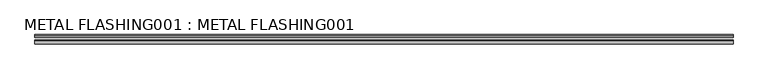
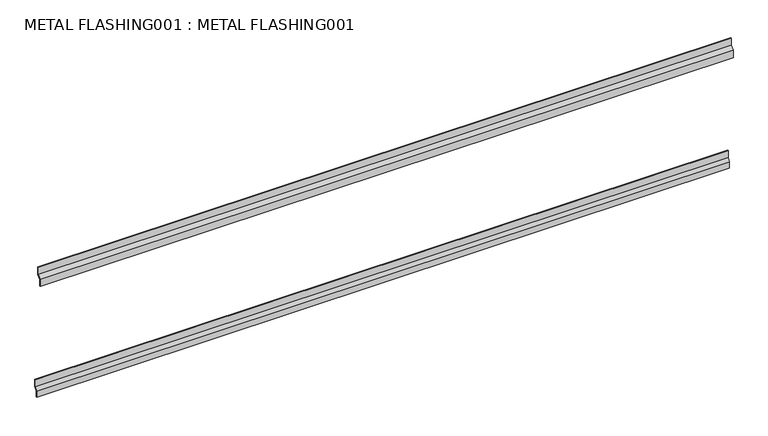
"""IFC4 building model written with IfcOpenShell, lengths in millimetres: proxy geometry, METAL FLASHING001 : METAL FLASHING001."""

import ifcopenshell
import ifcopenshell.guid

model = None  # the IFC model being written
_history = None  # IfcOwnerHistory: only IFC2X3 demands one
_inside = {}  # id of a spatial element -> (the spatial element, [elements in it])
_under = {}  # id of a project, library or spatial element -> (it, [spatial elements below it])
_declared = {}  # id of a project -> (the project, [libraries it declares])
_typed = {}  # id of a type object -> (the type object, [elements of that type])
_made_of = {}  # id of a material, layer set ... -> (it, [elements and type objects made of it])


def new_model(schema):
    """Start an empty IFC model of exactly this schema.

    Asked for "IFC4X3", IfcOpenShell would pick the latest addendum, in which some entities
    have other attributes; the version numbers below select the first issue.
    IFC2X3 requires an IfcOwnerHistory on every rooted entity: one is made here for all.
    """
    global model, _history
    if schema == "IFC4X3":
        model = ifcopenshell.file(schema_version=(4, 3, 0, 0))
    else:
        model = ifcopenshell.file(schema=schema)
    _inside.clear()
    _under.clear()
    _declared.clear()
    _typed.clear()
    _made_of.clear()
    _history = None
    if model.schema == "IFC2X3":
        org = make("IfcOrganization", Name="unknown")
        user = make(
            "IfcPersonAndOrganization",
            ThePerson=make("IfcPerson", FamilyName="unknown"),
            TheOrganization=org,
        )
        app = make(
            "IfcApplication",
            ApplicationDeveloper=org,
            Version="unknown",
            ApplicationFullName="unknown",
            ApplicationIdentifier="unknown",
        )
        _history = make(
            "IfcOwnerHistory",
            OwningUser=user,
            OwningApplication=app,
            ChangeAction="ADDED",
            CreationDate=0,
        )
    return model


def make(cls, **values):
    """One entity of the class cls with the attributes given. An attribute that is None is left unset."""
    return model.create_entity(
        cls, **{name: value for name, value in values.items() if value is not None}
    )


def rooted(cls, **values):
    """An entity with a GlobalId (a new one), such as an element, a storey or a relation."""
    return make(cls, GlobalId=ifcopenshell.guid.new(), OwnerHistory=_history, **values)


def si_unit(unit_type, name, prefix=None):
    """IfcSIUnit, for example si_unit("LENGTHUNIT", "METRE", prefix="MILLI")."""
    return make("IfcSIUnit", UnitType=unit_type, Prefix=prefix, Name=name)


def assignment(units):
    """IfcUnitAssignment: the units of a project."""
    return None if units is None else make("IfcUnitAssignment", Units=units)


def point(xyz):
    """IfcCartesianPoint."""
    return None if xyz is None else make("IfcCartesianPoint", Coordinates=xyz)


def direction(xyz):
    """IfcDirection."""
    return None if xyz is None else make("IfcDirection", DirectionRatios=xyz)


def frame(location, z_axis=None, x_axis=None):
    """IfcAxis2Placement3D, a coordinate frame: its origin and axes. An axis left out is left unset."""
    return make(
        "IfcAxis2Placement3D",
        Location=point(location),
        Axis=direction(z_axis),
        RefDirection=direction(x_axis),
    )


def origin():
    """The frame at (0, 0, 0) with its axes left unset."""
    return frame((0.0, 0.0, 0.0))


def place(relative_to, where):
    """IfcLocalPlacement: puts the frame where relative to a parent placement (None: the world)."""
    return make(
        "IfcLocalPlacement", PlacementRelTo=relative_to, RelativePlacement=where
    )


def context(
    kind, dimensions, precision=None, world=None, true_north=None, identifier=None
):
    """IfcGeometricRepresentationContext, for example the 3D "Model" context."""
    return make(
        "IfcGeometricRepresentationContext",
        ContextIdentifier=identifier,
        ContextType=kind,
        CoordinateSpaceDimension=dimensions,
        Precision=precision,
        WorldCoordinateSystem=world,
        TrueNorth=true_north,
    )


def project(units=None, contexts=None):
    """IfcProject with its units and contexts."""
    return rooted(
        "IfcProject",
        Name="project",
        RepresentationContexts=contexts,
        UnitsInContext=assignment(units),
    )


def spatial(cls, under=None, at=None, **own):
    """A site, building, storey or space (cls), placed at a placement, below another one or the project."""
    s = rooted(cls, ObjectPlacement=at, **own)
    if under is not None:
        _under.setdefault(under.id(), (under, []))[1].append(s)
    return s


def polyline(points):
    """IfcPolyline through the points."""
    return make("IfcPolyline", Points=[point(p) for p in points])


def outline(outer, holes=None, kind="AREA"):
    """IfcArbitraryClosedProfileDef: a profile drawn as a closed curve; with holes, ...WithVoids."""
    if holes is None:
        return make("IfcArbitraryClosedProfileDef", ProfileType=kind, OuterCurve=outer)
    return make(
        "IfcArbitraryProfileDefWithVoids",
        ProfileType=kind,
        OuterCurve=outer,
        InnerCurves=holes,
    )


def extrude(swept, where, along, depth):
    """IfcExtrudedAreaSolid: the profile swept, set in the frame where, extruded along a direction by depth."""
    return make(
        "IfcExtrudedAreaSolid",
        SweptArea=swept,
        Position=where,
        ExtrudedDirection=direction(along),
        Depth=depth,
    )


def shape(context_of_items, identifier, shape_type, items):
    """IfcShapeRepresentation: the items that make up one representation, for example the "Body"."""
    return make(
        "IfcShapeRepresentation",
        ContextOfItems=context_of_items,
        RepresentationIdentifier=identifier,
        RepresentationType=shape_type,
        Items=items,
    )


def source(mapping_origin, context_of_items, identifier, shape_type, items):
    """IfcRepresentationMap: a shape defined once, which mapped items show again and again."""
    return make(
        "IfcRepresentationMap",
        MappingOrigin=mapping_origin,
        MappedRepresentation=shape(context_of_items, identifier, shape_type, items),
    )


def transform(
    local_origin,
    x_axis=None,
    y_axis=None,
    z_axis=None,
    scale=None,
    scale2=None,
    scale3=None,
    uniform=True,
):
    """IfcCartesianTransformationOperator3D, or its non-uniform kind. x_axis, y_axis, z_axis: its Axis1, 2, 3."""
    if uniform:
        return make(
            "IfcCartesianTransformationOperator3D",
            Axis1=direction(x_axis),
            Axis2=direction(y_axis),
            LocalOrigin=point(local_origin),
            Scale=scale,
            Axis3=direction(z_axis),
        )
    return make(
        "IfcCartesianTransformationOperator3DnonUniform",
        Axis1=direction(x_axis),
        Axis2=direction(y_axis),
        LocalOrigin=point(local_origin),
        Scale=scale,
        Axis3=direction(z_axis),
        Scale2=scale2,
        Scale3=scale3,
    )


def mapped(mapping_source, mapping_target):
    """IfcMappedItem: shows the shape of a source again, moved by a transform."""
    return make(
        "IfcMappedItem", MappingSource=mapping_source, MappingTarget=mapping_target
    )


def made_of(thing, what):
    """Note that an element or type object is made of a material, layer set ...; save() writes the relation."""
    if what is not None:
        _made_of.setdefault(what.id(), (what, []))[1].append(thing)
    return thing


def element(
    cls,
    number,
    at=None,
    inside=None,
    cuts=None,
    type_object=None,
    material=None,
    context=None,
    identifier="Body",
    shape_type=None,
    held_by="IfcProductDefinitionShape",
    body=None,
    shapes=None,
    **own,
):
    """One element of the class cls, such as IfcWall. Its Tag is "e" and its number.

    at: its placement. inside: the storey or other place that contains it. cuts: it is an
    opening in that element (IfcRelVoidsElement). A single representation is given by context,
    identifier, shape_type and body (its items); several are given by shapes. held_by: the class
    of the entity that holds the representations. save() writes the other relations.
    """
    e = rooted(cls, Tag="e%d" % number, ObjectPlacement=at, **own)
    if body is not None:
        shapes = [shape(context, identifier, shape_type, body)]
    if shapes is not None:
        e.Representation = make(held_by, Representations=shapes)
    if inside is not None:
        _inside.setdefault(inside.id(), (inside, []))[1].append(e)
    if cuts is not None:
        rooted(
            "IfcRelVoidsElement", RelatingBuildingElement=cuts, RelatedOpeningElement=e
        )
    if type_object is not None:
        _typed.setdefault(type_object.id(), (type_object, []))[1].append(e)
    return made_of(e, material)


def aggregate(whole, parts):
    """IfcRelAggregates: a whole, such as a stair, and the parts it consists of."""
    return rooted("IfcRelAggregates", RelatingObject=whole, RelatedObjects=parts)


def save(model, path):
    """Write the relations noted so far, then the file.

    IfcRelAggregates (storeys below a building ...), IfcRelContainedInSpatialStructure (elements
    in a storey), IfcRelDefinesByType, IfcRelAssociatesMaterial and IfcRelDeclares: one each for
    every whole, place, type object, material and project.
    """
    for whole, parts in _under.values():
        aggregate(whole, parts)
    for where, things in _inside.values():
        rooted(
            "IfcRelContainedInSpatialStructure",
            RelatedElements=things,
            RelatingStructure=where,
        )
    for kind, things in _typed.values():
        rooted("IfcRelDefinesByType", RelatedObjects=things, RelatingType=kind)
    for what, things in _made_of.values():
        rooted("IfcRelAssociatesMaterial", RelatedObjects=things, RelatingMaterial=what)
    for by, libraries in _declared.values():
        rooted("IfcRelDeclares", RelatingContext=by, RelatedDefinitions=libraries)
    model.write(path)


def metal_flashing001_metal_flashing001_148fdf84(model_context):
    return source(origin(), model_context, "Body", "SweptSolid", [
        extrude(outline(polyline([(-5601.520996, 42709.570312), (-5611.268555, 42700.125), (-5611.268555, 42679.632812), (-5613.808555, 42679.632812), (-5613.808555, 42701.2006089), (-5604.060996, 42710.6459209), (-5604.060996, 42732.367188), (-5601.520996, 42732.367188), (-5601.520996, 42709.570312)])), frame((12382.7678845, 0.0, 0.0), z_axis=(1.0, 0.0, 0.0), x_axis=(0.0, 1.0, 0.0)), (0.0, 0.0, 1.0), 2000.25),
        extrude(outline(polyline([(-5586.8675368, 42358.078125), (-5592.980957, 42348.316406), (-5592.980957, 42330.03125), (-5595.520957, 42330.03125), (-5595.520957, 42349.0461179), (-5589.4075368, 42358.8078369), (-5589.4075368, 42380.582031), (-5586.8675368, 42380.582031), (-5586.8675368, 42358.078125)])), frame((12382.7678845, 0.0, 0.0), z_axis=(1.0, 0.0, 0.0), x_axis=(0.0, 1.0, 0.0)), (0.0, 0.0, 1.0), 2000.25),
    ])


if __name__ == "__main__":
    model = new_model("IFC4")
    model_context = context("Model", 3, world=origin())
    ifc_project = project(units=[si_unit("LENGTHUNIT", "METRE", prefix="MILLI")], contexts=[model_context])
    site = spatial("IfcSite", under=ifc_project)
    building = spatial("IfcBuilding", under=site)
    placement = place(None, origin())
    metal_flashing001_metal_flashing001_shape = metal_flashing001_metal_flashing001_148fdf84(model_context)
    element("IfcBuildingElementProxy", 1, Name="METAL FLASHING001 : METAL FLASHING001", ObjectType="METAL FLASHING001 : METAL FLASHING001", at=placement, inside=building, context=model_context, shape_type="MappedRepresentation", body=[
        mapped(metal_flashing001_metal_flashing001_shape, transform((0.0, 0.0, 0.0), x_axis=(1.0, 0.0, 0.0), y_axis=(0.0, 1.0, 0.0), z_axis=(0.0, 0.0, 1.0))),
    ])
    save(model, "model.ifc")

# Revit data of these elements
# Type "METAL FLASHING001 : METAL FLASHING001"
#   NameOverride = "METAL FLASHING001"
# Element 1 (IfcBuildingElementProxy, "METAL FLASHING001 : METAL FLASHING001")
#   Materials on its faces: "16 GA. COPPER BRAKE METAL FLASHING"
# Materials
#   "16 GA. COPPER BRAKE METAL FLASHING": class "Unassigned", colour RGB 128 128 128, transparency 0
